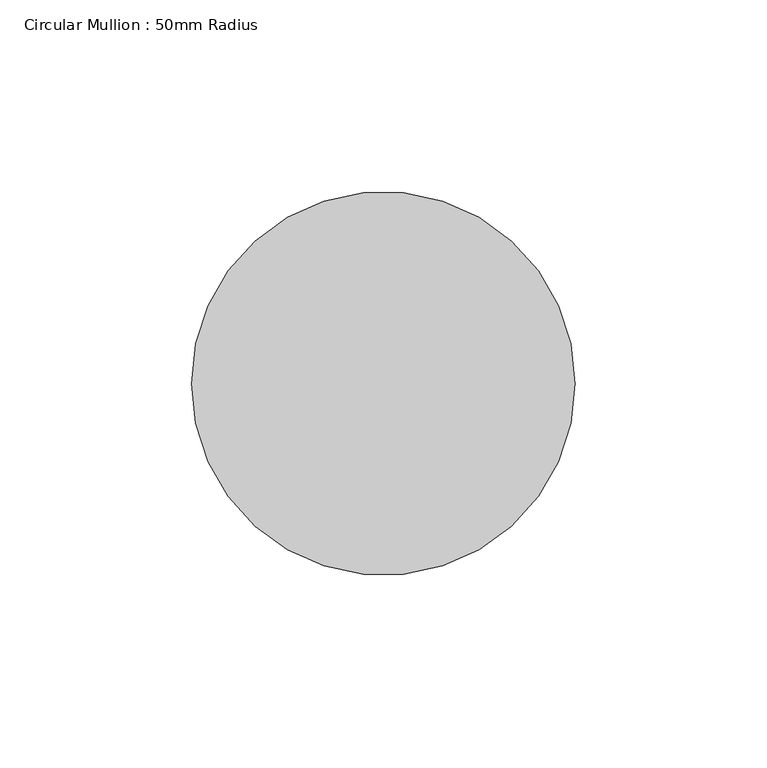
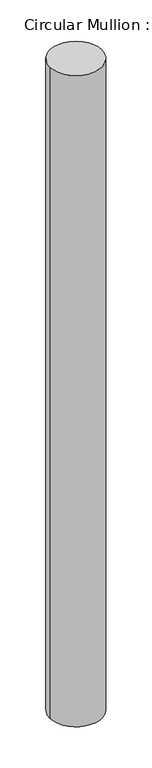
"""IFC4 building model written with IfcOpenShell, lengths in millimetres: member geometry, Circular Mullion : 50mm Radius."""

from ifc_helpers import new_model, si_unit, point, frame, origin, origin_2d, place, context, project, spatial, circle_curve, trimmed, segment, composite_curve, outline, extrude, source, transform, mapped, element, save


def circular_mullion_50mm_radius_8d69f96e(model_context):
    return source(origin(), model_context, "Body", "SweptSolid", [
        extrude(outline(composite_curve([segment(trimmed(circle_curve(origin_2d(), 50.0), [point((50.0, 0.0))], [point((-50.0, 0.0))], False, "CARTESIAN"), True, "CONTINUOUS"), segment(trimmed(circle_curve(origin_2d(), 50.0), [point((-50.0, 0.0))], [point((50.0, 0.0))], False, "CARTESIAN"), True, "CONTINUOUS")], self_intersect=False)), frame((0.0, 0.0, -1323.759907), z_axis=(0.0, 0.0, 1.0), x_axis=(1.0, 0.0, 0.0)), (0.0, 0.0, 1.0), 1323.759907),
    ])


if __name__ == "__main__":
    model = new_model("IFC4")
    model_context = context("Model", 3, world=origin())
    ifc_project = project(units=[si_unit("LENGTHUNIT", "METRE", prefix="MILLI")], contexts=[model_context])
    site = spatial("IfcSite", under=ifc_project)
    building = spatial("IfcBuilding", under=site)
    placement = place(None, origin())
    circular_mullion_50mm_radius_shape = circular_mullion_50mm_radius_8d69f96e(model_context)
    element("IfcMember", 1, ObjectType="Circular Mullion : 50mm Radius", at=placement, inside=building, context=model_context, shape_type="MappedRepresentation", body=[
        mapped(circular_mullion_50mm_radius_shape, transform((0.0, 0.0, 0.0), x_axis=(1.0, 0.0, 0.0), y_axis=(0.0, 1.0, 0.0), z_axis=(0.0, 0.0, 1.0))),
    ])
    save(model, "model.ifc")

# Revit data of these elements
# Type "Circular Mullion : 50mm Radius"
#   built-in parameter 1007350 = 0.164042 (stored number, unit not read)
# Element 1 (IfcMember, "Circular Mullion : 50mm Radius")
#   Materials on its faces: "Aluminium"
# Materials
#   "Aluminium": class "Metal", colour RGB 247 247 247, transparency 0, Description = "Aluminium 6061", Cost = 0
